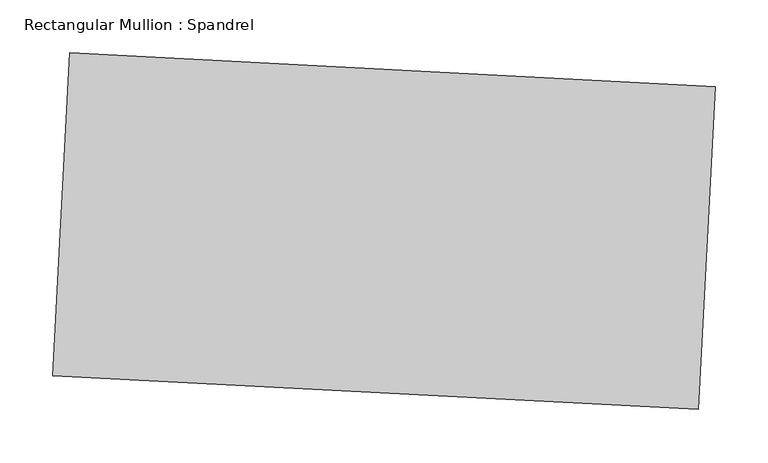
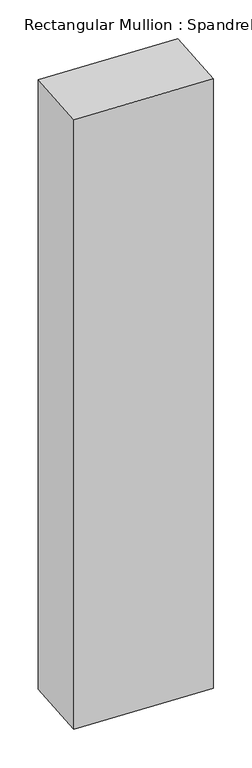
"""IFC4 building model written with IfcOpenShell, lengths in millimetres: member geometry, Rectangular Mullion : Spandrel."""

import ifcopenshell
import ifcopenshell.guid

model = None  # the IFC model being written
_history = None  # IfcOwnerHistory: only IFC2X3 demands one
_inside = {}  # id of a spatial element -> (the spatial element, [elements in it])
_under = {}  # id of a project, library or spatial element -> (it, [spatial elements below it])
_declared = {}  # id of a project -> (the project, [libraries it declares])
_typed = {}  # id of a type object -> (the type object, [elements of that type])
_made_of = {}  # id of a material, layer set ... -> (it, [elements and type objects made of it])


def new_model(schema):
    """Start an empty IFC model of exactly this schema.

    Asked for "IFC4X3", IfcOpenShell would pick the latest addendum, in which some entities
    have other attributes; the version numbers below select the first issue.
    IFC2X3 requires an IfcOwnerHistory on every rooted entity: one is made here for all.
    """
    global model, _history
    if schema == "IFC4X3":
        model = ifcopenshell.file(schema_version=(4, 3, 0, 0))
    else:
        model = ifcopenshell.file(schema=schema)
    _inside.clear()
    _under.clear()
    _declared.clear()
    _typed.clear()
    _made_of.clear()
    _history = None
    if model.schema == "IFC2X3":
        org = make("IfcOrganization", Name="unknown")
        user = make(
            "IfcPersonAndOrganization",
            ThePerson=make("IfcPerson", FamilyName="unknown"),
            TheOrganization=org,
        )
        app = make(
            "IfcApplication",
            ApplicationDeveloper=org,
            Version="unknown",
            ApplicationFullName="unknown",
            ApplicationIdentifier="unknown",
        )
        _history = make(
            "IfcOwnerHistory",
            OwningUser=user,
            OwningApplication=app,
            ChangeAction="ADDED",
            CreationDate=0,
        )
    return model


def make(cls, **values):
    """One entity of the class cls with the attributes given. An attribute that is None is left unset."""
    return model.create_entity(
        cls, **{name: value for name, value in values.items() if value is not None}
    )


def rooted(cls, **values):
    """An entity with a GlobalId (a new one), such as an element, a storey or a relation."""
    return make(cls, GlobalId=ifcopenshell.guid.new(), OwnerHistory=_history, **values)


def si_unit(unit_type, name, prefix=None):
    """IfcSIUnit, for example si_unit("LENGTHUNIT", "METRE", prefix="MILLI")."""
    return make("IfcSIUnit", UnitType=unit_type, Prefix=prefix, Name=name)


def assignment(units):
    """IfcUnitAssignment: the units of a project."""
    return None if units is None else make("IfcUnitAssignment", Units=units)


def point(xyz):
    """IfcCartesianPoint."""
    return None if xyz is None else make("IfcCartesianPoint", Coordinates=xyz)


def direction(xyz):
    """IfcDirection."""
    return None if xyz is None else make("IfcDirection", DirectionRatios=xyz)


def frame(location, z_axis=None, x_axis=None):
    """IfcAxis2Placement3D, a coordinate frame: its origin and axes. An axis left out is left unset."""
    return make(
        "IfcAxis2Placement3D",
        Location=point(location),
        Axis=direction(z_axis),
        RefDirection=direction(x_axis),
    )


def origin():
    """The frame at (0, 0, 0) with its axes left unset."""
    return frame((0.0, 0.0, 0.0))


def place(relative_to, where):
    """IfcLocalPlacement: puts the frame where relative to a parent placement (None: the world)."""
    return make(
        "IfcLocalPlacement", PlacementRelTo=relative_to, RelativePlacement=where
    )


def context(
    kind, dimensions, precision=None, world=None, true_north=None, identifier=None
):
    """IfcGeometricRepresentationContext, for example the 3D "Model" context."""
    return make(
        "IfcGeometricRepresentationContext",
        ContextIdentifier=identifier,
        ContextType=kind,
        CoordinateSpaceDimension=dimensions,
        Precision=precision,
        WorldCoordinateSystem=world,
        TrueNorth=true_north,
    )


def project(units=None, contexts=None):
    """IfcProject with its units and contexts."""
    return rooted(
        "IfcProject",
        Name="project",
        RepresentationContexts=contexts,
        UnitsInContext=assignment(units),
    )


def spatial(cls, under=None, at=None, **own):
    """A site, building, storey or space (cls), placed at a placement, below another one or the project."""
    s = rooted(cls, ObjectPlacement=at, **own)
    if under is not None:
        _under.setdefault(under.id(), (under, []))[1].append(s)
    return s


def polyline(points):
    """IfcPolyline through the points."""
    return make("IfcPolyline", Points=[point(p) for p in points])


def outline(outer, holes=None, kind="AREA"):
    """IfcArbitraryClosedProfileDef: a profile drawn as a closed curve; with holes, ...WithVoids."""
    if holes is None:
        return make("IfcArbitraryClosedProfileDef", ProfileType=kind, OuterCurve=outer)
    return make(
        "IfcArbitraryProfileDefWithVoids",
        ProfileType=kind,
        OuterCurve=outer,
        InnerCurves=holes,
    )


def extrude(swept, where, along, depth):
    """IfcExtrudedAreaSolid: the profile swept, set in the frame where, extruded along a direction by depth."""
    return make(
        "IfcExtrudedAreaSolid",
        SweptArea=swept,
        Position=where,
        ExtrudedDirection=direction(along),
        Depth=depth,
    )


def shape(context_of_items, identifier, shape_type, items):
    """IfcShapeRepresentation: the items that make up one representation, for example the "Body"."""
    return make(
        "IfcShapeRepresentation",
        ContextOfItems=context_of_items,
        RepresentationIdentifier=identifier,
        RepresentationType=shape_type,
        Items=items,
    )


def source(mapping_origin, context_of_items, identifier, shape_type, items):
    """IfcRepresentationMap: a shape defined once, which mapped items show again and again."""
    return make(
        "IfcRepresentationMap",
        MappingOrigin=mapping_origin,
        MappedRepresentation=shape(context_of_items, identifier, shape_type, items),
    )


def transform(
    local_origin,
    x_axis=None,
    y_axis=None,
    z_axis=None,
    scale=None,
    scale2=None,
    scale3=None,
    uniform=True,
):
    """IfcCartesianTransformationOperator3D, or its non-uniform kind. x_axis, y_axis, z_axis: its Axis1, 2, 3."""
    if uniform:
        return make(
            "IfcCartesianTransformationOperator3D",
            Axis1=direction(x_axis),
            Axis2=direction(y_axis),
            LocalOrigin=point(local_origin),
            Scale=scale,
            Axis3=direction(z_axis),
        )
    return make(
        "IfcCartesianTransformationOperator3DnonUniform",
        Axis1=direction(x_axis),
        Axis2=direction(y_axis),
        LocalOrigin=point(local_origin),
        Scale=scale,
        Axis3=direction(z_axis),
        Scale2=scale2,
        Scale3=scale3,
    )


def mapped(mapping_source, mapping_target):
    """IfcMappedItem: shows the shape of a source again, moved by a transform."""
    return make(
        "IfcMappedItem", MappingSource=mapping_source, MappingTarget=mapping_target
    )


def made_of(thing, what):
    """Note that an element or type object is made of a material, layer set ...; save() writes the relation."""
    if what is not None:
        _made_of.setdefault(what.id(), (what, []))[1].append(thing)
    return thing


def element(
    cls,
    number,
    at=None,
    inside=None,
    cuts=None,
    type_object=None,
    material=None,
    context=None,
    identifier="Body",
    shape_type=None,
    held_by="IfcProductDefinitionShape",
    body=None,
    shapes=None,
    **own,
):
    """One element of the class cls, such as IfcWall. Its Tag is "e" and its number.

    at: its placement. inside: the storey or other place that contains it. cuts: it is an
    opening in that element (IfcRelVoidsElement). A single representation is given by context,
    identifier, shape_type and body (its items); several are given by shapes. held_by: the class
    of the entity that holds the representations. save() writes the other relations.
    """
    e = rooted(cls, Tag="e%d" % number, ObjectPlacement=at, **own)
    if body is not None:
        shapes = [shape(context, identifier, shape_type, body)]
    if shapes is not None:
        e.Representation = make(held_by, Representations=shapes)
    if inside is not None:
        _inside.setdefault(inside.id(), (inside, []))[1].append(e)
    if cuts is not None:
        rooted(
            "IfcRelVoidsElement", RelatingBuildingElement=cuts, RelatedOpeningElement=e
        )
    if type_object is not None:
        _typed.setdefault(type_object.id(), (type_object, []))[1].append(e)
    return made_of(e, material)


def aggregate(whole, parts):
    """IfcRelAggregates: a whole, such as a stair, and the parts it consists of."""
    return rooted("IfcRelAggregates", RelatingObject=whole, RelatedObjects=parts)


def save(model, path):
    """Write the relations noted so far, then the file.

    IfcRelAggregates (storeys below a building ...), IfcRelContainedInSpatialStructure (elements
    in a storey), IfcRelDefinesByType, IfcRelAssociatesMaterial and IfcRelDeclares: one each for
    every whole, place, type object, material and project.
    """
    for whole, parts in _under.values():
        aggregate(whole, parts)
    for where, things in _inside.values():
        rooted(
            "IfcRelContainedInSpatialStructure",
            RelatedElements=things,
            RelatingStructure=where,
        )
    for kind, things in _typed.values():
        rooted("IfcRelDefinesByType", RelatedObjects=things, RelatingType=kind)
    for what, things in _made_of.values():
        rooted("IfcRelAssociatesMaterial", RelatedObjects=things, RelatingMaterial=what)
    for by, libraries in _declared.values():
        rooted("IfcRelDeclares", RelatingContext=by, RelatedDefinitions=libraries)
    model.write(path)


def rectangular_mullion_spandrel_ef47994c(model_context):
    return source(origin(), model_context, "Body", "SweptSolid", [
        extrude(outline(polyline([(7.5582819, 136.2391416), (-8.3937175, -168.1431406), (-617.1582819, -136.2391416), (-601.2062825, 168.1431406), (7.5582819, 136.2391416)])), frame((0.0, 0.0, -2900.7036942), z_axis=(0.0, 0.0, 1.0), x_axis=(1.0, 0.0, 0.0)), (0.0, 0.0, 1.0), 2900.7036942),
    ])


if __name__ == "__main__":
    model = new_model("IFC4")
    model_context = context("Model", 3, world=origin())
    ifc_project = project(units=[si_unit("LENGTHUNIT", "METRE", prefix="MILLI")], contexts=[model_context])
    site = spatial("IfcSite", under=ifc_project)
    building = spatial("IfcBuilding", under=site)
    placement = place(None, origin())
    rectangular_mullion_spandrel_shape = rectangular_mullion_spandrel_ef47994c(model_context)
    element("IfcMember", 1, ObjectType="Rectangular Mullion : Spandrel", at=placement, inside=building, context=model_context, shape_type="MappedRepresentation", body=[
        mapped(rectangular_mullion_spandrel_shape, transform((0.0, 0.0, 0.0), x_axis=(1.0, 0.0, 0.0), y_axis=(0.0, 1.0, 0.0), z_axis=(0.0, 0.0, 1.0))),
    ])
    save(model, "model.ifc")

# Revit data of these elements
# Type "Rectangular Mullion : Spandrel"
#   built-in parameter 1007304 = 1 (stored number, unit not read)
#   built-in parameter 1007301 = 1 (stored number, unit not read)
#   built-in parameter 1007300 = 1 (stored number, unit not read)
# Element 1 (IfcMember, "Rectangular Mullion : Spandrel")
#   Materials on its faces: "Aluminum"
# Materials
#   "Aluminum": class "Metal", colour RGB 247 247 247, transparency 0, Description = "Aluminum 6061", Cost = 0
